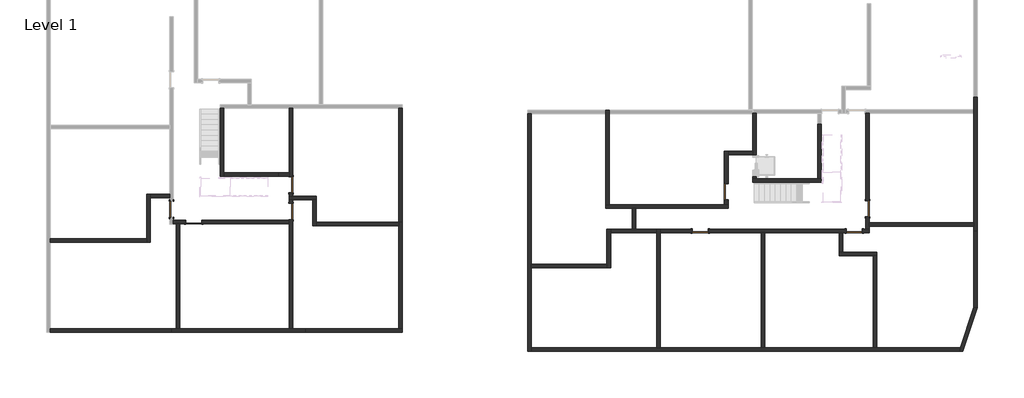
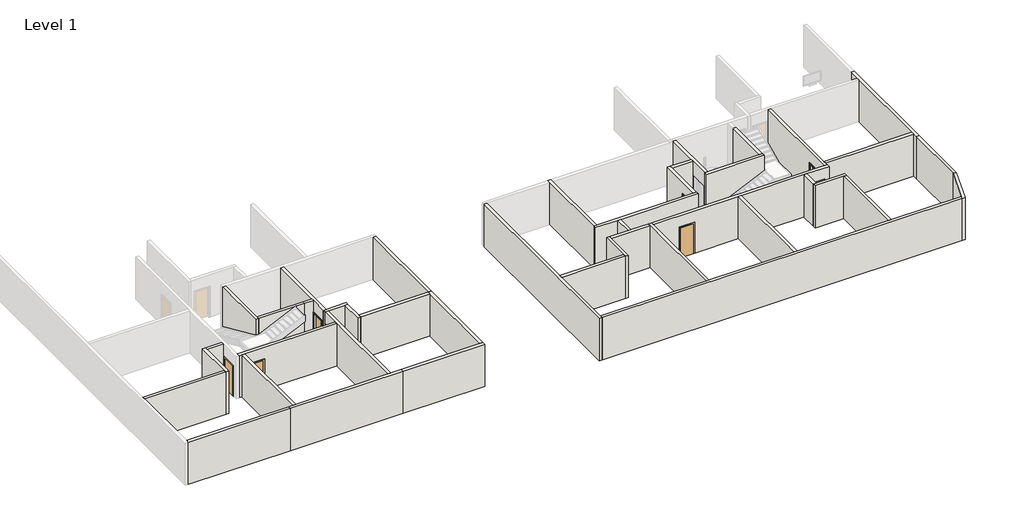
# One storey, part 1 of 2: 42 walls, 8 doors.
"""IFC4 building model written with IfcOpenShell, lengths in millimetres."""

import ifcopenshell
import ifcopenshell.guid

model = None  # the IFC model being written
_history = None  # IfcOwnerHistory: only IFC2X3 demands one
_inside = {}  # id of a spatial element -> (the spatial element, [elements in it])
_under = {}  # id of a project, library or spatial element -> (it, [spatial elements below it])
_declared = {}  # id of a project -> (the project, [libraries it declares])
_typed = {}  # id of a type object -> (the type object, [elements of that type])
_made_of = {}  # id of a material, layer set ... -> (it, [elements and type objects made of it])


def new_model(schema):
    """Start an empty IFC model of exactly this schema.

    Asked for "IFC4X3", IfcOpenShell would pick the latest addendum, in which some entities
    have other attributes; the version numbers below select the first issue.
    IFC2X3 requires an IfcOwnerHistory on every rooted entity: one is made here for all.
    """
    global model, _history
    if schema == "IFC4X3":
        model = ifcopenshell.file(schema_version=(4, 3, 0, 0))
    else:
        model = ifcopenshell.file(schema=schema)
    _inside.clear()
    _under.clear()
    _declared.clear()
    _typed.clear()
    _made_of.clear()
    _history = None
    if model.schema == "IFC2X3":
        org = make("IfcOrganization", Name="unknown")
        user = make(
            "IfcPersonAndOrganization",
            ThePerson=make("IfcPerson", FamilyName="unknown"),
            TheOrganization=org,
        )
        app = make(
            "IfcApplication",
            ApplicationDeveloper=org,
            Version="unknown",
            ApplicationFullName="unknown",
            ApplicationIdentifier="unknown",
        )
        _history = make(
            "IfcOwnerHistory",
            OwningUser=user,
            OwningApplication=app,
            ChangeAction="ADDED",
            CreationDate=0,
        )
    return model


def make(cls, **values):
    """One entity of the class cls with the attributes given. An attribute that is None is left unset."""
    return model.create_entity(
        cls, **{name: value for name, value in values.items() if value is not None}
    )


def rooted(cls, **values):
    """An entity with a GlobalId (a new one), such as an element, a storey or a relation."""
    return make(cls, GlobalId=ifcopenshell.guid.new(), OwnerHistory=_history, **values)


def si_unit(unit_type, name, prefix=None):
    """IfcSIUnit, for example si_unit("LENGTHUNIT", "METRE", prefix="MILLI")."""
    return make("IfcSIUnit", UnitType=unit_type, Prefix=prefix, Name=name)


def assignment(units):
    """IfcUnitAssignment: the units of a project."""
    return None if units is None else make("IfcUnitAssignment", Units=units)


def point(xyz):
    """IfcCartesianPoint."""
    return None if xyz is None else make("IfcCartesianPoint", Coordinates=xyz)


def direction(xyz):
    """IfcDirection."""
    return None if xyz is None else make("IfcDirection", DirectionRatios=xyz)


def frame(location, z_axis=None, x_axis=None):
    """IfcAxis2Placement3D, a coordinate frame: its origin and axes. An axis left out is left unset."""
    return make(
        "IfcAxis2Placement3D",
        Location=point(location),
        Axis=direction(z_axis),
        RefDirection=direction(x_axis),
    )


def origin():
    """The frame at (0, 0, 0) with its axes left unset."""
    return frame((0.0, 0.0, 0.0))


def origin_with_axes():
    """The frame at (0, 0, 0) with the z axis (0, 0, 1) and the x axis (1, 0, 0) written out."""
    return frame((0.0, 0.0, 0.0), z_axis=(0.0, 0.0, 1.0), x_axis=(1.0, 0.0, 0.0))


def place(relative_to, where):
    """IfcLocalPlacement: puts the frame where relative to a parent placement (None: the world)."""
    return make(
        "IfcLocalPlacement", PlacementRelTo=relative_to, RelativePlacement=where
    )


def context(
    kind, dimensions, precision=None, world=None, true_north=None, identifier=None
):
    """IfcGeometricRepresentationContext, for example the 3D "Model" context."""
    return make(
        "IfcGeometricRepresentationContext",
        ContextIdentifier=identifier,
        ContextType=kind,
        CoordinateSpaceDimension=dimensions,
        Precision=precision,
        WorldCoordinateSystem=world,
        TrueNorth=true_north,
    )


def project(units=None, contexts=None):
    """IfcProject with its units and contexts."""
    return rooted(
        "IfcProject",
        Name="project",
        RepresentationContexts=contexts,
        UnitsInContext=assignment(units),
    )


def spatial(cls, under=None, at=None, **own):
    """A site, building, storey or space (cls), placed at a placement, below another one or the project."""
    s = rooted(cls, ObjectPlacement=at, **own)
    if under is not None:
        _under.setdefault(under.id(), (under, []))[1].append(s)
    return s


def polyline(points):
    """IfcPolyline through the points."""
    return make("IfcPolyline", Points=[point(p) for p in points])


def outline(outer, holes=None, kind="AREA"):
    """IfcArbitraryClosedProfileDef: a profile drawn as a closed curve; with holes, ...WithVoids."""
    if holes is None:
        return make("IfcArbitraryClosedProfileDef", ProfileType=kind, OuterCurve=outer)
    return make(
        "IfcArbitraryProfileDefWithVoids",
        ProfileType=kind,
        OuterCurve=outer,
        InnerCurves=holes,
    )


def extrude(swept, where, along, depth):
    """IfcExtrudedAreaSolid: the profile swept, set in the frame where, extruded along a direction by depth."""
    return make(
        "IfcExtrudedAreaSolid",
        SweptArea=swept,
        Position=where,
        ExtrudedDirection=direction(along),
        Depth=depth,
    )


def faces_of(points, faces, orient=None, outer=None):
    """IfcFace entities. A face is a list of loops; a loop is a list of indices into points, from 0.

    orient and outer hold one flag for each loop. By default every Orientation is true, the
    first loop of a face is its IfcFaceOuterBound and the others are IfcFaceBound.
    """
    made = []
    for i, loops in enumerate(faces):
        bounds = []
        for j, loop in enumerate(loops):
            is_outer = j == 0 if outer is None else outer[i][j]
            bounds.append(
                make(
                    "IfcFaceOuterBound" if is_outer else "IfcFaceBound",
                    Bound=make("IfcPolyLoop", Polygon=[points[k] for k in loop]),
                    Orientation=True if orient is None else orient[i][j],
                )
            )
        made.append(make("IfcFace", Bounds=bounds))
    return made


def faceted_brep(points, faces, orient=None, outer=None, voids=None):
    """IfcFacetedBrep: a solid bounded by flat faces; with voids (closed shells), ...WithVoids."""
    shared = [point(p) for p in points]
    hull = make("IfcClosedShell", CfsFaces=faces_of(shared, faces, orient, outer))
    if voids is None:
        return make("IfcFacetedBrep", Outer=hull)
    return make(
        "IfcFacetedBrepWithVoids",
        Outer=hull,
        Voids=[
            make(cls, CfsFaces=faces_of(shared, fs, o, b)) for cls, fs, o, b in voids
        ],
    )


def shape(context_of_items, identifier, shape_type, items):
    """IfcShapeRepresentation: the items that make up one representation, for example the "Body"."""
    return make(
        "IfcShapeRepresentation",
        ContextOfItems=context_of_items,
        RepresentationIdentifier=identifier,
        RepresentationType=shape_type,
        Items=items,
    )


def source(mapping_origin, context_of_items, identifier, shape_type, items):
    """IfcRepresentationMap: a shape defined once, which mapped items show again and again."""
    return make(
        "IfcRepresentationMap",
        MappingOrigin=mapping_origin,
        MappedRepresentation=shape(context_of_items, identifier, shape_type, items),
    )


def transform(
    local_origin,
    x_axis=None,
    y_axis=None,
    z_axis=None,
    scale=None,
    scale2=None,
    scale3=None,
    uniform=True,
):
    """IfcCartesianTransformationOperator3D, or its non-uniform kind. x_axis, y_axis, z_axis: its Axis1, 2, 3."""
    if uniform:
        return make(
            "IfcCartesianTransformationOperator3D",
            Axis1=direction(x_axis),
            Axis2=direction(y_axis),
            LocalOrigin=point(local_origin),
            Scale=scale,
            Axis3=direction(z_axis),
        )
    return make(
        "IfcCartesianTransformationOperator3DnonUniform",
        Axis1=direction(x_axis),
        Axis2=direction(y_axis),
        LocalOrigin=point(local_origin),
        Scale=scale,
        Axis3=direction(z_axis),
        Scale2=scale2,
        Scale3=scale3,
    )


def mapped(mapping_source, mapping_target):
    """IfcMappedItem: shows the shape of a source again, moved by a transform."""
    return make(
        "IfcMappedItem", MappingSource=mapping_source, MappingTarget=mapping_target
    )


def made_of(thing, what):
    """Note that an element or type object is made of a material, layer set ...; save() writes the relation."""
    if what is not None:
        _made_of.setdefault(what.id(), (what, []))[1].append(thing)
    return thing


def element(
    cls,
    number,
    at=None,
    inside=None,
    cuts=None,
    type_object=None,
    material=None,
    context=None,
    identifier="Body",
    shape_type=None,
    held_by="IfcProductDefinitionShape",
    body=None,
    shapes=None,
    **own,
):
    """One element of the class cls, such as IfcWall. Its Tag is "e" and its number.

    at: its placement. inside: the storey or other place that contains it. cuts: it is an
    opening in that element (IfcRelVoidsElement). A single representation is given by context,
    identifier, shape_type and body (its items); several are given by shapes. held_by: the class
    of the entity that holds the representations. save() writes the other relations.
    """
    e = rooted(cls, Tag="e%d" % number, ObjectPlacement=at, **own)
    if body is not None:
        shapes = [shape(context, identifier, shape_type, body)]
    if shapes is not None:
        e.Representation = make(held_by, Representations=shapes)
    if inside is not None:
        _inside.setdefault(inside.id(), (inside, []))[1].append(e)
    if cuts is not None:
        rooted(
            "IfcRelVoidsElement", RelatingBuildingElement=cuts, RelatedOpeningElement=e
        )
    if type_object is not None:
        _typed.setdefault(type_object.id(), (type_object, []))[1].append(e)
    return made_of(e, material)


def aggregate(whole, parts):
    """IfcRelAggregates: a whole, such as a stair, and the parts it consists of."""
    return rooted("IfcRelAggregates", RelatingObject=whole, RelatedObjects=parts)


def save(model, path):
    """Write the relations noted so far, then the file.

    IfcRelAggregates (storeys below a building ...), IfcRelContainedInSpatialStructure (elements
    in a storey), IfcRelDefinesByType, IfcRelAssociatesMaterial and IfcRelDeclares: one each for
    every whole, place, type object, material and project.
    """
    for whole, parts in _under.values():
        aggregate(whole, parts)
    for where, things in _inside.values():
        rooted(
            "IfcRelContainedInSpatialStructure",
            RelatedElements=things,
            RelatingStructure=where,
        )
    for kind, things in _typed.values():
        rooted("IfcRelDefinesByType", RelatedObjects=things, RelatingType=kind)
    for what, things in _made_of.values():
        rooted("IfcRelAssociatesMaterial", RelatedObjects=things, RelatingMaterial=what)
    for by, libraries in _declared.values():
        rooted("IfcRelDeclares", RelatingContext=by, RelatedDefinitions=libraries)
    model.write(path)


def m_single_flush_0915_x_2134mm_727434cd(model_context):
    return source(origin(), model_context, "Body", "SweptSolid", [
        extrude(outline(polyline([(2210.0, -533.5), (0.0, -533.5), (0.0, -457.5), (2134.0, -457.5), (2134.0, 457.5), (0.0, 457.5), (0.0, 533.5), (2210.0, 533.5), (2210.0, -533.5)])), frame((0.0, -125.0, 0.0), z_axis=(0.0, 1.0, 0.0), x_axis=(0.0, 0.0, 1.0)), (0.0, 0.0, 1.0), 25.0),
        extrude(outline(polyline([(2210.0, 533.5), (2210.0, -533.5), (0.0, -533.5), (0.0, -457.5), (2134.0, -457.5), (2134.0, 457.5), (0.0, 457.5), (0.0, 533.5), (2210.0, 533.5)])), frame((0.0, 100.0, 0.0), z_axis=(0.0, 1.0, 0.0), x_axis=(0.0, 0.0, 1.0)), (0.0, 0.0, 1.0), 25.0),
        extrude(outline(polyline([(457.5, -49.0), (457.5, -100.0), (-457.5, -100.0), (-457.5, -49.0), (457.5, -49.0)])), origin_with_axes(), (0.0, 0.0, 1.0), 2134.0),
    ])


def m_single_flush_0915_x_2134mm_6a9e8738(model_context):
    return source(origin(), model_context, "Body", "SweptSolid", [
        extrude(outline(polyline([(2210.0, -533.5), (0.0, -533.5), (0.0, -457.5), (2134.0, -457.5), (2134.0, 457.5), (0.0, 457.5), (0.0, 533.5), (2210.0, 533.5), (2210.0, -533.5)])), frame((0.0, 100.0, 0.0), z_axis=(0.0, 1.0, 0.0), x_axis=(0.0, 0.0, 1.0)), (0.0, 0.0, 1.0), 25.0),
        extrude(outline(polyline([(2210.0, 533.5), (2210.0, -533.5), (0.0, -533.5), (0.0, -457.5), (2134.0, -457.5), (2134.0, 457.5), (0.0, 457.5), (0.0, 533.5), (2210.0, 533.5)])), frame((0.0, -125.0, 0.0), z_axis=(0.0, 1.0, 0.0), x_axis=(0.0, 0.0, 1.0)), (0.0, 0.0, 1.0), 25.0),
        extrude(outline(polyline([(457.5, 49.0), (-457.5, 49.0), (-457.5, 100.0), (457.5, 100.0), (457.5, 49.0)])), origin_with_axes(), (0.0, 0.0, 1.0), 2134.0),
    ])


model = new_model("IFC4")

# Units and contexts
model_context = context("Model", 3, world=origin())
ifc_project = project(units=[si_unit("LENGTHUNIT", "METRE", prefix="MILLI")], contexts=[model_context])

# Site, building, storey
site = spatial("IfcSite", under=ifc_project)
building = spatial("IfcBuilding", under=site)
storey = spatial("IfcBuildingStorey", under=building, Name="Level 1", Elevation=0.0)

# Doors
placement = place(None, origin())
m_single_flush_0915_x_2134mm_shape = m_single_flush_0915_x_2134mm_727434cd(model_context)
element("IfcDoor", 1, ObjectType="M_Single-Flush : 0915 x 2134mm", at=placement, inside=storey, context=model_context, shape_type="MappedRepresentation", body=[
    mapped(m_single_flush_0915_x_2134mm_shape, transform((16070.6041014, -3023.024372, 0.0), x_axis=(0.0, -1.0, 0.0), y_axis=(1.0, 0.0, 0.0), z_axis=(0.0, 0.0, 1.0))),
])
element("IfcDoor", 2, ObjectType="M_Single-Flush : 0915 x 2134mm", at=placement, inside=storey, context=model_context, shape_type="MappedRepresentation", body=[
    mapped(m_single_flush_0915_x_2134mm_shape, transform((-8530.3449834, -4137.6378151, 0.0), x_axis=(0.0, 1.0, 0.0), y_axis=(-1.0, 0.0, 0.0), z_axis=(0.0, 0.0, 1.0))),
])
m_single_flush_0915_x_2134mm_2_shape = m_single_flush_0915_x_2134mm_6a9e8738(model_context)
element("IfcDoor", 3, ObjectType="M_Single-Flush : 0915 x 2134mm", at=placement, inside=storey, context=model_context, shape_type="MappedRepresentation", body=[
    mapped(m_single_flush_0915_x_2134mm_2_shape, transform((14602.336337, -5240.0098119, 0.0), x_axis=(-1.0, 0.0, 0.0), y_axis=(0.0, -1.0, 0.0), z_axis=(0.0, 0.0, 1.0))),
])
element("IfcDoor", 4, ObjectType="M_Single-Flush : 0915 x 2134mm", at=placement, inside=storey, context=model_context, shape_type="MappedRepresentation", body=[
    mapped(m_single_flush_0915_x_2134mm_2_shape, transform((24048.8612349, -3982.5098119, 0.0), x_axis=(0.0, -1.0, 0.0), y_axis=(1.0, 0.0, 0.0), z_axis=(0.0, 0.0, 1.0))),
])
element("IfcDoor", 5, ObjectType="M_Single-Flush : 0915 x 2134mm", at=placement, inside=storey, context=model_context, shape_type="MappedRepresentation", body=[
    mapped(m_single_flush_0915_x_2134mm_2_shape, transform((23308.8612349, -5240.0098119, 0.0), x_axis=(-1.0, 0.0, 0.0), y_axis=(0.0, -1.0, 0.0), z_axis=(0.0, 0.0, 1.0))),
])
element("IfcDoor", 6, ObjectType="M_Single-Flush : 0915 x 2134mm", at=placement, inside=storey, context=model_context, shape_type="MappedRepresentation", body=[
    mapped(m_single_flush_0915_x_2134mm_2_shape, transform((-14032.3304233, -4739.1627129, 0.0), x_axis=(-1.0, 0.0, 0.0), y_axis=(0.0, -1.0, 0.0), z_axis=(0.0, 0.0, 1.0))),
])
element("IfcDoor", 7, ObjectType="M_Single-Flush : 0915 x 2134mm", at=placement, inside=storey, context=model_context, shape_type="MappedRepresentation", body=[
    mapped(m_single_flush_0915_x_2134mm_2_shape, transform((-8530.3449834, -2622.6378151, 0.0), x_axis=(0.0, -1.0, 0.0), y_axis=(1.0, 0.0, 0.0), z_axis=(0.0, 0.0, 1.0))),
])
element("IfcDoor", 8, ObjectType="M_Single-Flush : 0915 x 2134mm", at=placement, inside=storey, context=model_context, shape_type="MappedRepresentation", body=[
    mapped(m_single_flush_0915_x_2134mm_2_shape, transform((-15289.8304233, -3999.1627129, 0.0), x_axis=(0.0, 1.0, 0.0), y_axis=(-1.0, 0.0, 0.0), z_axis=(0.0, 0.0, 1.0))),
])

# Walls
element("IfcWall", 9, ObjectType="Generic - 200mm", at=placement, inside=storey, context=model_context, shape_type="Brep", body=[
    faceted_brep([(30068.8612349, 2319.475628, 0.0), (30068.8612349, 1619.475628, 0.0), (30068.8612349, 1419.475628, 0.0), (30068.8612349, -4760.0098119, 0.0), (30068.8612349, -4960.0098119, 0.0), (30068.8612349, -5240.0098119, 0.0), (30068.8612349, -5240.0098119, 3000.0), (30068.8612349, -4960.0098119, 3000.0), (30068.8612349, -4760.0098119, 3000.0), (30068.8612349, 1419.475628, 3000.0), (30068.8612349, 1619.475628, 3000.0), (30068.8612349, 2319.475628, 3000.0), (30268.8612349, 2319.475628, 0.0), (30268.8612349, 2319.475628, 3000.0), (30268.8612349, -5240.0098119, 3000.0), (30268.8612349, -5240.0098119, 0.0), (30268.3425199, 2319.475628, 0.0), (30069.3799498, -5240.0098119, 0.0), (30069.3799498, -5240.0098119, 3000.0), (30268.3425199, 2319.475628, 3000.0)], [[[0, 1, 2, 3, 4, 5, 6, 7, 8, 9, 10, 11]], [[12, 13, 14, 15]], [[5, 4, 3, 2, 1, 0, 16, 12, 15, 17]], [[6, 5, 17, 15, 14, 18]], [[11, 10, 9, 8, 7, 6, 18, 14, 13, 19]], [[0, 11, 19, 13, 12, 16]]]),
])
element("IfcWall", 10, ObjectType="Generic - 200mm", at=placement, inside=storey, context=model_context, shape_type="Brep", body=[
    faceted_brep([(30069.3799498, -5240.0098119, 0.0), (30069.3799498, -9543.0251929, 0.0), (30069.3799498, -9543.0251929, 3000.0), (30069.3799498, -5240.0098119, 3000.0), (30269.3799498, -5240.0098119, 0.0), (30269.3799498, -5240.0098119, 3000.0), (30269.3799498, -9575.863443, 3000.0), (30269.3799498, -9575.863443, 0.0), (30268.8612349, -5240.0098119, 0.0), (30268.8612349, -5240.0098119, 3000.0)], [[[0, 1, 2, 3]], [[4, 5, 6, 7]], [[1, 0, 8, 4, 7]], [[3, 2, 6, 5, 9]], [[0, 3, 9, 5, 4, 8]], [[2, 1, 7, 6]]]),
])
element("IfcWall", 11, ObjectType="Generic - 200mm", at=placement, inside=storey, context=model_context, shape_type="Brep", body=[
    faceted_brep([(21449.836337, -2276.2808257, 0.0), (21249.836337, -2276.2808257, 0.0), (17770.6041014, -2276.2808257, 0.0), (17570.6041014, -2276.2808257, 0.0), (17570.6041014, -2276.2808257, 3000.0), (17770.6041014, -2276.2808257, 3000.0), (21249.836337, -2276.2808257, 3000.0), (21449.836337, -2276.2808257, 3000.0), (21449.836337, -2476.2808257, 0.0), (21449.836337, -2476.2808257, 3000.0), (17570.6041014, -2476.2808257, 3000.0), (17570.6041014, -2476.2808257, 0.0)], [[[0, 1, 2, 3, 4, 5, 6, 7]], [[8, 9, 10, 11]], [[3, 2, 1, 0, 8, 11]], [[7, 6, 5, 4, 10, 9]], [[0, 7, 9, 8]], [[4, 3, 11, 10]]]),
])
element("IfcWall", 12, ObjectType="Generic - 200mm", at=placement, inside=storey, context=model_context, shape_type="SweptSolid", body=[
    extrude(outline(polyline([(18259.836337, -5340.0098119), (18259.836337, -11836.6907835), (18059.836337, -11836.6907835), (18059.836337, -5340.0098119), (18259.836337, -5340.0098119)])), origin_with_axes(), (0.0, 0.0, 1.0), 3000.0),
])
element("IfcWall", 13, ObjectType="Generic - 200mm", at=placement, inside=storey, context=model_context, shape_type="Brep", body=[
    faceted_brep([(29295.3124022, -11836.6907835, 0.0), (24588.8612349, -11836.6907835, 0.0), (24388.8612349, -11836.6907835, 0.0), (18259.836337, -11836.6907835, 0.0), (18059.836337, -11836.6907835, 0.0), (12342.1281129, -11836.6907835, 0.0), (12142.1281129, -11836.6907835, 0.0), (5043.716007, -11836.6907835, 0.0), (5043.716007, -11836.6907835, 3000.0), (12142.1281129, -11836.6907835, 3000.0), (12342.1281129, -11836.6907835, 3000.0), (18059.836337, -11836.6907835, 3000.0), (18259.836337, -11836.6907835, 3000.0), (24388.8612349, -11836.6907835, 3000.0), (24588.8612349, -11836.6907835, 3000.0), (29295.3124022, -11836.6907835, 3000.0), (29227.8162902, -12036.6907835, 0.0), (29227.8162902, -12036.6907835, 3000.0), (5043.716007, -12036.6907835, 3000.0), (5043.716007, -12036.6907835, 0.0)], [[[0, 1, 2, 3, 4, 5, 6, 7, 8, 9, 10, 11, 12, 13, 14, 15]], [[16, 17, 18, 19]], [[7, 6, 5, 4, 3, 2, 1, 0, 16, 19]], [[15, 14, 13, 12, 11, 10, 9, 8, 18, 17]], [[0, 15, 17, 16]], [[8, 7, 19, 18]]]),
])
element("IfcWall", 14, ObjectType="Generic - 200mm", at=placement, inside=storey, context=model_context, shape_type="Brep", body=[
    faceted_brep([(30069.3799498, -9543.0251929, 0.0), (29295.3124022, -11836.6907835, 0.0), (29227.8162902, -12036.6907835, 0.0), (29227.8162902, -12036.6907835, 3000.0), (29295.3124022, -11836.6907835, 3000.0), (30069.3799498, -9543.0251929, 3000.0), (30269.3799498, -9575.863443, 0.0), (30269.3799498, -9575.863443, 3000.0), (29438.8985612, -12036.6907835, 3000.0), (29438.8985612, -12036.6907835, 0.0)], [[[0, 1, 2, 3, 4, 5]], [[6, 7, 8, 9]], [[2, 1, 0, 6, 9]], [[5, 4, 3, 8, 7]], [[0, 5, 7, 6]], [[3, 2, 9, 8]]]),
])
element("IfcWall", 15, ObjectType="Generic - 200mm", at=placement, inside=storey, context=model_context, shape_type="Brep", body=[
    faceted_brep([(22851.3612349, -5140.0098119, 2134.0), (22851.3612349, -5140.0098119, 0.0), (15059.836337, -5140.0098119, 0.0), (15059.836337, -5140.0098119, 2134.0), (14144.836337, -5140.0098119, 2134.0), (14144.836337, -5140.0098119, 0.0), (12342.1281129, -5140.0098119, 0.0), (12342.1281129, -5140.0098119, 3000.0), (23948.8612349, -5140.0098119, 3000.0), (24148.8612349, -5140.0098119, 3000.0), (24163.3998354, -5140.0098119, 3000.0), (24163.3998354, -5140.0098119, 0.0), (24148.8612349, -5140.0098119, 0.0), (23948.8612349, -5140.0098119, 0.0), (23766.3612349, -5140.0098119, 0.0), (23766.3612349, -5140.0098119, 2134.0), (15059.836337, -5340.0098119, 0.0), (18059.836337, -5340.0098119, 0.0), (18259.836337, -5340.0098119, 0.0), (22468.8612349, -5340.0098119, 0.0), (22668.8612349, -5340.0098119, 0.0), (22851.3612349, -5340.0098119, 0.0), (22851.3612349, -5340.0098119, 2134.0), (23766.3612349, -5340.0098119, 2134.0), (23766.3612349, -5340.0098119, 0.0), (24163.3998354, -5340.0098119, 0.0), (24163.3998354, -5340.0098119, 3000.0), (22668.8612349, -5340.0098119, 3000.0), (22468.8612349, -5340.0098119, 3000.0), (18259.836337, -5340.0098119, 3000.0), (18059.836337, -5340.0098119, 3000.0), (12342.1281129, -5340.0098119, 3000.0), (12342.1281129, -5340.0098119, 0.0), (14144.836337, -5340.0098119, 0.0), (14144.836337, -5340.0098119, 2134.0), (15059.836337, -5340.0098119, 2134.0)], [[[0, 1, 2, 3, 4, 5, 6, 7, 8, 9, 10, 11, 12, 13, 14, 15]], [[16, 17, 18, 19, 20, 21, 22, 23, 24, 25, 26, 27, 28, 29, 30, 31, 32, 33, 34, 35]], [[32, 6, 5, 33]], [[2, 1, 21, 20, 19, 18, 17, 16]], [[14, 13, 12, 11, 25, 24]], [[10, 9, 8, 7, 31, 30, 29, 28, 27, 26]], [[11, 10, 26, 25]], [[4, 34, 33, 5]], [[35, 3, 2, 16]], [[3, 35, 34, 4]], [[22, 21, 1, 0]], [[23, 22, 0, 15]], [[24, 23, 15, 14]], [[7, 6, 32, 31]]]),
])
element("IfcWall", 16, ObjectType="Generic - 200mm", at=placement, inside=storey, context=model_context, shape_type="Brep", body=[
    faceted_brep([(4843.716007, 1379.9901881, 0.0), (4843.716007, -12036.6907835, 0.0), (4843.716007, -12036.6907835, 3000.0), (4843.716007, 1379.9901881, 3000.0), (5043.716007, 1379.9901881, 0.0), (5043.716007, 1379.9901881, 3000.0), (5043.716007, -7120.0098119, 3000.0), (5043.716007, -7320.0098119, 3000.0), (5043.716007, -11836.6907835, 3000.0), (5043.716007, -12036.6907835, 3000.0), (5043.716007, -12036.6907835, 0.0), (5043.716007, -11836.6907835, 0.0), (5043.716007, -7320.0098119, 0.0), (5043.716007, -7120.0098119, 0.0)], [[[0, 1, 2, 3]], [[4, 5, 6, 7, 8, 9, 10, 11, 12, 13]], [[1, 0, 4, 13, 12, 11, 10]], [[3, 2, 9, 8, 7, 6, 5]], [[2, 1, 10, 9]], [[0, 3, 5, 4]]]),
])
element("IfcWall", 17, ObjectType="Generic - 200mm", at=placement, inside=storey, context=model_context, shape_type="Brep", body=[
    faceted_brep([(24148.8612349, 1419.475628, 3000.0), (24148.8612349, -4760.0098119, 3000.0), (24148.8612349, -4960.0098119, 3000.0), (24148.8612349, -5140.0098119, 3000.0), (24148.8612349, -5140.0098119, 0.0), (24148.8612349, -4960.0098119, 0.0), (24148.8612349, -4760.0098119, 0.0), (24148.8612349, -4440.0098119, 0.0), (24148.8612349, -4440.0098119, 2134.0), (24148.8612349, -3525.0098119, 2134.0), (24148.8612349, -3525.0098119, 0.0), (24148.8612349, 1419.475628, 0.0), (23948.8612349, -5140.0098119, 3000.0), (23948.8612349, 1419.475628, 3000.0), (23948.8612349, 1419.475628, 0.0), (23948.8612349, -3525.0098119, 0.0), (23948.8612349, -3525.0098119, 2134.0), (23948.8612349, -4440.0098119, 2134.0), (23948.8612349, -4440.0098119, 0.0), (23948.8612349, -5140.0098119, 0.0)], [[[0, 1, 2, 3, 4, 5, 6, 7, 8, 9, 10, 11]], [[12, 13, 14, 15, 16, 17, 18, 19]], [[14, 11, 10, 15]], [[4, 19, 18, 7, 6, 5]], [[3, 2, 1, 0, 13, 12]], [[0, 11, 14, 13]], [[17, 8, 7, 18]], [[9, 16, 15, 10]], [[16, 9, 8, 17]], [[4, 3, 12, 19]]]),
])
element("IfcWall", 18, ObjectType="Generic - 200mm", at=placement, inside=storey, context=model_context, shape_type="SweptSolid", body=[
    extrude(outline(polyline([(21249.836337, -2276.2808257), (21249.836337, 799.475628), (21449.836337, 799.475628), (21449.836337, -2276.2808257), (21249.836337, -2276.2808257)])), origin_with_axes(), (0.0, 0.0, 1.0), 3000.0),
])
element("IfcWall", 19, ObjectType="Generic - 200mm", at=placement, inside=storey, context=model_context, shape_type="Brep", body=[
    faceted_brep([(17570.6041014, -2276.2808257, 3000.0), (17570.6041014, -920.524372, 3000.0), (17570.6041014, -720.524372, 3000.0), (17570.6041014, 1379.475628, 3000.0), (17570.6041014, 1419.475628, 3000.0), (17570.6041014, 1419.475628, 0.0), (17570.6041014, 1379.475628, 0.0), (17570.6041014, -720.524372, 0.0), (17570.6041014, -920.524372, 0.0), (17570.6041014, -926.2808257, 0.0), (17570.6041014, -926.2808257, 2000.0), (17570.6041014, -2181.2876228, 2000.0), (17570.6041014, -2181.2876228, 0.0), (17570.6041014, -2276.2808257, 0.0), (17770.6041014, 1419.475628, 3000.0), (17770.6041014, -2276.2808257, 3000.0), (17770.6041014, -2276.2808257, 0.0), (17770.6041014, -2181.2876228, 0.0), (17770.6041014, -2181.2876228, 2000.0), (17770.6041014, -926.2808257, 2000.0), (17770.6041014, -926.2808257, 0.0), (17770.6041014, 1419.475628, 0.0)], [[[0, 1, 2, 3, 4, 5, 6, 7, 8, 9, 10, 11, 12, 13]], [[14, 15, 16, 17, 18, 19, 20, 21]], [[16, 13, 12, 17]], [[5, 21, 20, 9, 8, 7, 6]], [[4, 3, 2, 1, 0, 15, 14]], [[0, 13, 16, 15]], [[5, 4, 14, 21]], [[11, 18, 17, 12]], [[19, 10, 9, 20]], [[10, 19, 18, 11]]]),
])
element("IfcWall", 20, ObjectType="Generic - 200mm", at=placement, inside=storey, context=model_context, shape_type="Brep", body=[
    faceted_brep([(9268.8612349, -3940.0098119, 0.0), (10768.8612349, -3940.0098119, 0.0), (10968.8612349, -3940.0098119, 0.0), (16170.6041014, -3940.0098119, 0.0), (16170.6041014, -3940.0098119, 3000.0), (10968.8612349, -3940.0098119, 3000.0), (10768.8612349, -3940.0098119, 3000.0), (9268.8612349, -3940.0098119, 3000.0), (9268.8612349, -3740.0098119, 0.0), (9268.8612349, -3740.0098119, 3000.0), (9468.8612349, -3740.0098119, 3000.0), (15970.6041014, -3740.0098119, 3000.0), (16170.6041014, -3740.0098119, 3000.0), (16170.6041014, -3740.0098119, 0.0), (15970.6041014, -3740.0098119, 0.0), (9468.8612349, -3740.0098119, 0.0)], [[[0, 1, 2, 3, 4, 5, 6, 7]], [[8, 9, 10, 11, 12, 13, 14, 15]], [[3, 2, 1, 0, 8, 15, 14, 13]], [[7, 6, 5, 4, 12, 11, 10, 9]], [[4, 3, 13, 12]], [[0, 7, 9, 8]]]),
])
element("IfcWall", 21, ObjectType="Generic - 200mm", at=placement, inside=storey, context=model_context, shape_type="Brep", body=[
    faceted_brep([(16170.6041014, -720.524372, 3000.0), (16170.6041014, -920.524372, 3000.0), (16170.6041014, -3740.0098119, 3000.0), (16170.6041014, -3740.0098119, 0.0), (16170.6041014, -3480.524372, 0.0), (16170.6041014, -3480.524372, 2134.0), (16170.6041014, -2565.524372, 2134.0), (16170.6041014, -2565.524372, 0.0), (16170.6041014, -920.524372, 0.0), (16170.6041014, -720.524372, 0.0), (15970.6041014, -3740.0098119, 3000.0), (15970.6041014, -720.524372, 3000.0), (15970.6041014, -720.524372, 0.0), (15970.6041014, -2565.524372, 0.0), (15970.6041014, -2565.524372, 2134.0), (15970.6041014, -3480.524372, 2134.0), (15970.6041014, -3480.524372, 0.0), (15970.6041014, -3740.0098119, 0.0)], [[[0, 1, 2, 3, 4, 5, 6, 7, 8, 9]], [[10, 11, 12, 13, 14, 15, 16, 17]], [[3, 17, 16, 4]], [[12, 9, 8, 7, 13]], [[2, 1, 0, 11, 10]], [[3, 2, 10, 17]], [[0, 9, 12, 11]], [[15, 5, 4, 16]], [[6, 14, 13, 7]], [[14, 6, 5, 15]]]),
])
element("IfcWall", 22, ObjectType="Generic - 200mm", at=placement, inside=storey, context=model_context, shape_type="SweptSolid", body=[
    extrude(outline(polyline([(17570.6041014, -920.524372), (16170.6041014, -920.524372), (16170.6041014, -720.524372), (17570.6041014, -720.524372), (17570.6041014, -920.524372)])), origin_with_axes(), (0.0, 0.0, 1.0), 3000.0),
])
element("IfcWall", 23, ObjectType="Generic - 200mm", at=placement, inside=storey, context=model_context, shape_type="Brep", body=[
    faceted_brep([(22468.8612349, -6641.2808257, 0.0), (24388.8612349, -6641.2808257, 0.0), (24588.8612349, -6641.2808257, 0.0), (24588.8612349, -6641.2808257, 3000.0), (24388.8612349, -6641.2808257, 3000.0), (22468.8612349, -6641.2808257, 3000.0), (22468.8612349, -6441.2808257, 0.0), (22468.8612349, -6441.2808257, 3000.0), (22668.8612349, -6441.2808257, 3000.0), (24588.8612349, -6441.2808257, 3000.0), (24588.8612349, -6441.2808257, 0.0), (22668.8612349, -6441.2808257, 0.0)], [[[0, 1, 2, 3, 4, 5]], [[6, 7, 8, 9, 10, 11]], [[2, 1, 0, 6, 11, 10]], [[5, 4, 3, 9, 8, 7]], [[3, 2, 10, 9]], [[0, 5, 7, 6]]]),
])
element("IfcWall", 24, ObjectType="Generic - 200mm", at=placement, inside=storey, context=model_context, shape_type="SweptSolid", body=[
    extrude(outline(polyline([(24388.8612349, -11836.6907835), (24388.8612349, -6641.2808257), (24588.8612349, -6641.2808257), (24588.8612349, -11836.6907835), (24388.8612349, -11836.6907835)])), origin_with_axes(), (0.0, 0.0, 1.0), 3000.0),
])
element("IfcWall", 25, ObjectType="Generic - 200mm", at=placement, inside=storey, context=model_context, shape_type="SweptSolid", body=[
    extrude(outline(polyline([(22668.8612349, -5340.0098119), (22668.8612349, -6441.2808257), (22468.8612349, -6441.2808257), (22468.8612349, -5340.0098119), (22668.8612349, -5340.0098119)])), origin_with_axes(), (0.0, 0.0, 1.0), 3000.0),
])
element("IfcWall", 26, ObjectType="Generic - 200mm", at=placement, inside=storey, context=model_context, shape_type="SweptSolid", body=[
    extrude(outline(polyline([(30068.8612349, -4960.0098119), (24148.8612349, -4960.0098119), (24148.8612349, -4760.0098119), (30068.8612349, -4760.0098119), (30068.8612349, -4960.0098119)])), origin_with_axes(), (0.0, 0.0, 1.0), 3000.0),
])
element("IfcWall", 27, ObjectType="Generic - 200mm", at=placement, inside=storey, context=model_context, shape_type="Brep", body=[
    faceted_brep([(9268.8612349, 1579.9901881, 0.0), (9268.8612349, 1379.9901881, 0.0), (9268.8612349, -3740.0098119, 0.0), (9268.8612349, -3740.0098119, 3000.0), (9268.8612349, 1379.9901881, 3000.0), (9268.8612349, 1579.9901881, 3000.0), (9468.8612349, 1579.9901881, 0.0), (9468.8612349, 1579.9901881, 3000.0), (9468.8612349, 1579.475628, 3000.0), (9468.8612349, 1379.475628, 3000.0), (9468.8612349, -3740.0098119, 3000.0), (9468.8612349, -3740.0098119, 0.0), (9468.8612349, 1379.475628, 0.0), (9468.8612349, 1579.475628, 0.0)], [[[0, 1, 2, 3, 4, 5]], [[6, 7, 8, 9, 10, 11, 12, 13]], [[2, 1, 0, 6, 13, 12, 11]], [[5, 4, 3, 10, 9, 8, 7]], [[3, 2, 11, 10]], [[0, 5, 7, 6]]]),
])
element("IfcWall", 28, ObjectType="Generic - 200mm", at=placement, inside=storey, context=model_context, shape_type="SweptSolid", body=[
    extrude(outline(polyline([(5043.716007, -7120.0098119), (9328.8612349, -7120.0098119), (9328.8612349, -7320.0098119), (5043.716007, -7320.0098119), (5043.716007, -7120.0098119)])), origin_with_axes(), (0.0, 0.0, 1.0), 3000.0),
])
element("IfcWall", 29, ObjectType="Generic - 200mm", at=placement, inside=storey, context=model_context, shape_type="Brep", body=[
    faceted_brep([(-2430.3449834, -4740.1378151, 0.0), (-2430.3449834, -4940.1378151, 0.0), (-2430.3449834, -10758.643998, 0.0), (-2430.3449834, -10758.643998, 3000.0), (-2430.3449834, -4940.1378151, 3000.0), (-2430.3449834, -4740.1378151, 3000.0), (-2230.3449834, -4740.1378151, 0.0), (-2230.3449834, -4740.1378151, 3000.0), (-2230.3449834, -10758.643998, 3000.0), (-2230.3449834, -10758.643998, 0.0)], [[[0, 1, 2, 3, 4, 5]], [[6, 7, 8, 9]], [[2, 1, 0, 6, 9]], [[5, 4, 3, 8, 7]], [[3, 2, 9, 8]], [[0, 5, 7, 6]]]),
])
element("IfcWall", 30, ObjectType="Generic - 200mm", at=placement, inside=storey, context=model_context, shape_type="Brep", body=[
    faceted_brep([(-2230.3449834, -10758.643998, 0.0), (-2430.3449834, -10758.643998, 0.0), (-7730.3449834, -10758.643998, 0.0), (-7730.3449834, -10758.643998, 3000.0), (-2430.3449834, -10758.643998, 3000.0), (-2230.3449834, -10758.643998, 3000.0), (-2230.3449834, -10958.643998, 0.0), (-2230.3449834, -10958.643998, 3000.0), (-7730.3449834, -10958.643998, 3000.0), (-7730.3449834, -10958.643998, 0.0), (-7730.3449834, -10759.1627129, 0.0), (-7730.3449834, -10759.1627129, 3000.0)], [[[0, 1, 2, 3, 4, 5]], [[6, 7, 8, 9]], [[2, 1, 0, 6, 9, 10]], [[3, 2, 10, 9, 8, 11]], [[5, 4, 3, 11, 8, 7]], [[0, 5, 7, 6]]]),
])
element("IfcWall", 31, ObjectType="Generic - 200mm", at=placement, inside=storey, context=model_context, shape_type="Brep", body=[
    faceted_brep([(-7730.3449834, -10759.1627129, 0.0), (-8430.3449834, -10759.1627129, 0.0), (-8630.3449834, -10759.1627129, 0.0), (-14809.8304233, -10759.1627129, 0.0), (-15009.8304233, -10759.1627129, 0.0), (-15289.8304233, -10759.1627129, 0.0), (-15289.8304233, -10759.1627129, 3000.0), (-15009.8304233, -10759.1627129, 3000.0), (-14809.8304233, -10759.1627129, 3000.0), (-8630.3449834, -10759.1627129, 3000.0), (-8430.3449834, -10759.1627129, 3000.0), (-7730.3449834, -10759.1627129, 3000.0), (-7730.3449834, -10959.1627129, 0.0), (-7730.3449834, -10959.1627129, 3000.0), (-15289.8304233, -10959.1627129, 3000.0), (-15289.8304233, -10959.1627129, 0.0), (-7730.3449834, -10958.643998, 0.0), (-15289.8304233, -10759.6814279, 0.0), (-15289.8304233, -10759.6814279, 3000.0), (-7730.3449834, -10958.643998, 3000.0)], [[[0, 1, 2, 3, 4, 5, 6, 7, 8, 9, 10, 11]], [[12, 13, 14, 15]], [[5, 4, 3, 2, 1, 0, 16, 12, 15, 17]], [[6, 5, 17, 15, 14, 18]], [[11, 10, 9, 8, 7, 6, 18, 14, 13, 19]], [[0, 11, 19, 13, 12, 16]]]),
])
element("IfcWall", 32, ObjectType="Generic - 200mm", at=placement, inside=storey, context=model_context, shape_type="Brep", body=[
    faceted_brep([(-15289.8304233, -10759.6814279, 0.0), (-22146.5113948, -10759.6814279, 0.0), (-22146.5113948, -10759.6814279, 3000.0), (-15289.8304233, -10759.6814279, 3000.0), (-15289.8304233, -10959.6814279, 0.0), (-15289.8304233, -10959.6814279, 3000.0), (-22146.5113948, -10959.6814279, 3000.0), (-22146.5113948, -10959.6814279, 0.0), (-15289.8304233, -10959.1627129, 0.0), (-15289.8304233, -10959.1627129, 3000.0)], [[[0, 1, 2, 3]], [[4, 5, 6, 7]], [[1, 0, 8, 4, 7]], [[3, 2, 6, 5, 9]], [[0, 3, 9, 5, 4, 8]], [[2, 1, 7, 6]]]),
])
element("IfcWall", 33, ObjectType="Generic - 200mm", at=placement, inside=storey, context=model_context, shape_type="Brep", body=[
    faceted_brep([(-12326.101437, -2140.1378151, 0.0), (-12326.101437, -1940.1378151, 0.0), (-12326.101437, 1699.0944206, 0.0), (-12326.101437, 1699.0944206, 3000.0), (-12326.101437, -1940.1378151, 3000.0), (-12326.101437, -2140.1378151, 3000.0), (-12526.101437, -2140.1378151, 0.0), (-12526.101437, -2140.1378151, 3000.0), (-12526.101437, 1699.0944206, 3000.0), (-12526.101437, 1699.0944206, 0.0)], [[[0, 1, 2, 3, 4, 5]], [[6, 7, 8, 9]], [[2, 1, 0, 6, 9]], [[3, 2, 9, 8]], [[5, 4, 3, 8, 7]], [[0, 5, 7, 6]]]),
])
element("IfcWall", 34, ObjectType="Generic - 200mm", at=placement, inside=storey, context=model_context, shape_type="Brep", body=[
    faceted_brep([(-8630.3449834, -4839.1627129, 3000.0), (-14809.8304233, -4839.1627129, 3000.0), (-15009.8304233, -4839.1627129, 3000.0), (-15189.8304233, -4839.1627129, 3000.0), (-15189.8304233, -4839.1627129, 0.0), (-15009.8304233, -4839.1627129, 0.0), (-14809.8304233, -4839.1627129, 0.0), (-14489.8304233, -4839.1627129, 0.0), (-14489.8304233, -4839.1627129, 2134.0), (-13574.8304233, -4839.1627129, 2134.0), (-13574.8304233, -4839.1627129, 0.0), (-8630.3449834, -4839.1627129, 0.0), (-15189.8304233, -4639.1627129, 3000.0), (-8630.3449834, -4639.1627129, 3000.0), (-8630.3449834, -4639.1627129, 0.0), (-13574.8304233, -4639.1627129, 0.0), (-13574.8304233, -4639.1627129, 2134.0), (-14489.8304233, -4639.1627129, 2134.0), (-14489.8304233, -4639.1627129, 0.0), (-15189.8304233, -4639.1627129, 0.0)], [[[0, 1, 2, 3, 4, 5, 6, 7, 8, 9, 10, 11]], [[12, 13, 14, 15, 16, 17, 18, 19]], [[14, 11, 10, 15]], [[4, 19, 18, 7, 6, 5]], [[3, 2, 1, 0, 13, 12]], [[0, 11, 14, 13]], [[17, 8, 7, 18]], [[9, 16, 15, 10]], [[16, 9, 8, 17]], [[4, 3, 12, 19]]]),
])
element("IfcWall", 35, ObjectType="Generic - 200mm", at=placement, inside=storey, context=model_context, shape_type="SweptSolid", body=[
    extrude(outline(polyline([(-12326.101437, -1940.1378151), (-9250.3449834, -1940.1378151), (-9250.3449834, -2140.1378151), (-12326.101437, -2140.1378151), (-12326.101437, -1940.1378151)])), origin_with_axes(), (0.0, 0.0, 1.0), 3000.0),
])
element("IfcWall", 36, ObjectType="Generic - 200mm", at=placement, inside=storey, context=model_context, shape_type="SweptSolid", body=[
    extrude(outline(polyline([(-8630.3449834, -2140.1378151), (-9250.3449834, -2140.1378151), (-9250.3449834, -1940.1378151), (-8630.3449834, -1940.1378151), (-8630.3449834, -2140.1378151)])), origin_with_axes(), (0.0, 0.0, 1.0), 3000.0),
])
element("IfcWall", 37, ObjectType="Generic - 200mm", at=placement, inside=storey, context=model_context, shape_type="SweptSolid", body=[
    extrude(outline(polyline([(-2430.3449834, -4740.1378151), (-2430.3449834, 1700.8372871), (-2230.3449834, 1700.8372871), (-2230.3449834, -4740.1378151), (-2430.3449834, -4740.1378151)])), origin_with_axes(), (0.0, 0.0, 1.0), 3000.0),
])
element("IfcWall", 38, ObjectType="Generic - 200mm", at=placement, inside=storey, context=model_context, shape_type="Brep", body=[
    faceted_brep([(-8630.3449834, -3480.1378151, 0.0), (-8430.3449834, -3480.1378151, 0.0), (-7295.3449834, -3480.1378151, 0.0), (-7095.3449834, -3480.1378151, 0.0), (-7095.3449834, -3480.1378151, 3000.0), (-7295.3449834, -3480.1378151, 3000.0), (-8430.3449834, -3480.1378151, 3000.0), (-8630.3449834, -3480.1378151, 3000.0), (-8630.3449834, -3280.1378151, 0.0), (-8630.3449834, -3280.1378151, 3000.0), (-8430.3449834, -3280.1378151, 3000.0), (-7095.3449834, -3280.1378151, 3000.0), (-7095.3449834, -3280.1378151, 0.0), (-8430.3449834, -3280.1378151, 0.0)], [[[0, 1, 2, 3, 4, 5, 6, 7]], [[8, 9, 10, 11, 12, 13]], [[3, 2, 1, 0, 8, 13, 12]], [[7, 6, 5, 4, 11, 10, 9]], [[0, 7, 9, 8]], [[4, 3, 12, 11]]]),
])
element("IfcWall", 39, ObjectType="Generic - 200mm", at=placement, inside=storey, context=model_context, shape_type="Brep", body=[
    faceted_brep([(-8630.3449834, -10759.1627129, 3000.0), (-8630.3449834, -4839.1627129, 3000.0), (-8630.3449834, -4639.1627129, 3000.0), (-8630.3449834, -3480.1378151, 3000.0), (-8630.3449834, -3480.1378151, 0.0), (-8630.3449834, -3680.1378151, 0.0), (-8630.3449834, -3680.1378151, 2134.0), (-8630.3449834, -4595.1378151, 2134.0), (-8630.3449834, -4595.1378151, 0.0), (-8630.3449834, -4639.1627129, 0.0), (-8630.3449834, -4839.1627129, 0.0), (-8630.3449834, -10759.1627129, 0.0), (-8430.3449834, -3480.1378151, 3000.0), (-8430.3449834, -10759.1627129, 3000.0), (-8430.3449834, -10759.1627129, 0.0), (-8430.3449834, -4595.1378151, 0.0), (-8430.3449834, -4595.1378151, 2134.0), (-8430.3449834, -3680.1378151, 2134.0), (-8430.3449834, -3680.1378151, 0.0), (-8430.3449834, -3480.1378151, 0.0)], [[[0, 1, 2, 3, 4, 5, 6, 7, 8, 9, 10, 11]], [[12, 13, 14, 15, 16, 17, 18, 19]], [[14, 11, 10, 9, 8, 15]], [[4, 19, 18, 5]], [[3, 2, 1, 0, 13, 12]], [[0, 11, 14, 13]], [[4, 3, 12, 19]], [[17, 6, 5, 18]], [[7, 16, 15, 8]], [[16, 7, 6, 17]]]),
])
element("IfcWall", 40, ObjectType="Generic - 200mm", at=placement, inside=storey, context=model_context, shape_type="Brep", body=[
    faceted_brep([(-8430.3449834, 1700.8372871, 3000.0), (-8430.3449834, -3280.1378151, 3000.0), (-8430.3449834, -3280.1378151, 0.0), (-8430.3449834, -3080.1378151, 0.0), (-8430.3449834, -3080.1378151, 2134.0), (-8430.3449834, -2165.1378151, 2134.0), (-8430.3449834, -2165.1378151, 0.0), (-8430.3449834, 1700.8372871, 0.0), (-8630.3449834, -3280.1378151, 3000.0), (-8630.3449834, -2140.1378151, 3000.0), (-8630.3449834, -1940.1378151, 3000.0), (-8630.3449834, 1700.8372871, 3000.0), (-8630.3449834, 1700.8372871, 0.0), (-8630.3449834, -1940.1378151, 0.0), (-8630.3449834, -2140.1378151, 0.0), (-8630.3449834, -2165.1378151, 0.0), (-8630.3449834, -2165.1378151, 2134.0), (-8630.3449834, -3080.1378151, 2134.0), (-8630.3449834, -3080.1378151, 0.0), (-8630.3449834, -3280.1378151, 0.0)], [[[0, 1, 2, 3, 4, 5, 6, 7]], [[8, 9, 10, 11, 12, 13, 14, 15, 16, 17, 18, 19]], [[2, 19, 18, 3]], [[12, 7, 6, 15, 14, 13]], [[1, 0, 11, 10, 9, 8]], [[2, 1, 8, 19]], [[17, 4, 3, 18]], [[5, 16, 15, 6]], [[16, 5, 4, 17]], [[0, 7, 12, 11]]]),
])
element("IfcWall", 41, ObjectType="Generic - 200mm", at=placement, inside=storey, context=model_context, shape_type="Brep", body=[
    faceted_brep([(-7295.3449834, -3480.1378151, 0.0), (-7295.3449834, -4940.1378151, 0.0), (-7295.3449834, -4940.1378151, 3000.0), (-7295.3449834, -3480.1378151, 3000.0), (-7095.3449834, -3480.1378151, 0.0), (-7095.3449834, -3480.1378151, 3000.0), (-7095.3449834, -4740.1378151, 3000.0), (-7095.3449834, -4940.1378151, 3000.0), (-7095.3449834, -4940.1378151, 0.0), (-7095.3449834, -4740.1378151, 0.0)], [[[0, 1, 2, 3]], [[4, 5, 6, 7, 8, 9]], [[1, 0, 4, 9, 8]], [[3, 2, 7, 6, 5]], [[2, 1, 8, 7]], [[0, 3, 5, 4]]]),
])
element("IfcWall", 42, ObjectType="Generic - 200mm", at=placement, inside=storey, context=model_context, shape_type="SweptSolid", body=[
    extrude(outline(polyline([(-2430.3449834, -4940.1378151), (-7095.3449834, -4940.1378151), (-7095.3449834, -4740.1378151), (-2430.3449834, -4740.1378151), (-2430.3449834, -4940.1378151)])), origin_with_axes(), (0.0, 0.0, 1.0), 3000.0),
])
element("IfcWall", 43, ObjectType="Generic - 200mm", at=placement, inside=storey, context=model_context, shape_type="Brep", body=[
    faceted_brep([(-16691.101437, -3159.1627129, 0.0), (-16691.101437, -5679.1627129, 0.0), (-16691.101437, -5879.1627129, 0.0), (-16691.101437, -5879.1627129, 3000.0), (-16691.101437, -5679.1627129, 3000.0), (-16691.101437, -3159.1627129, 3000.0), (-16491.101437, -3159.1627129, 0.0), (-16491.101437, -3159.1627129, 3000.0), (-16491.101437, -3359.1627129, 3000.0), (-16491.101437, -5879.1627129, 3000.0), (-16491.101437, -5879.1627129, 0.0), (-16491.101437, -3359.1627129, 0.0)], [[[0, 1, 2, 3, 4, 5]], [[6, 7, 8, 9, 10, 11]], [[2, 1, 0, 6, 11, 10]], [[5, 4, 3, 9, 8, 7]], [[3, 2, 10, 9]], [[0, 5, 7, 6]]]),
])
element("IfcWall", 44, ObjectType="Generic - 200mm", at=placement, inside=storey, context=model_context, shape_type="SweptSolid", body=[
    extrude(outline(polyline([(-22146.5113948, -5679.1627129), (-16691.101437, -5679.1627129), (-16691.101437, -5879.1627129), (-22146.5113948, -5879.1627129), (-22146.5113948, -5679.1627129)])), origin_with_axes(), (0.0, 0.0, 1.0), 3000.0),
])
element("IfcWall", 45, ObjectType="Generic - 200mm", at=placement, inside=storey, context=model_context, shape_type="SweptSolid", body=[
    extrude(outline(polyline([(-15389.8304233, -3359.1627129), (-16491.101437, -3359.1627129), (-16491.101437, -3159.1627129), (-15389.8304233, -3159.1627129), (-15389.8304233, -3359.1627129)])), origin_with_axes(), (0.0, 0.0, 1.0), 3000.0),
])
element("IfcWall", 46, ObjectType="Generic - 200mm", at=placement, inside=storey, context=model_context, shape_type="SweptSolid", body=[
    extrude(outline(polyline([(-15009.8304233, -10759.1627129), (-15009.8304233, -4839.1627129), (-14809.8304233, -4839.1627129), (-14809.8304233, -10759.1627129), (-15009.8304233, -10759.1627129)])), origin_with_axes(), (0.0, 0.0, 1.0), 3000.0),
])
element("IfcWall", 47, ObjectType="Generic - 200mm", at=placement, inside=storey, context=model_context, shape_type="Brep", body=[
    faceted_brep([(12142.1281129, -5136.6907835, 0.0), (12142.1281129, -5336.6907835, 0.0), (12142.1281129, -11836.6907835, 0.0), (12142.1281129, -11836.6907835, 3000.0), (12142.1281129, -5336.6907835, 3000.0), (12142.1281129, -5136.6907835, 3000.0), (12342.1281129, -5136.6907835, 0.0), (12342.1281129, -5136.6907835, 3000.0), (12342.1281129, -5140.0098119, 3000.0), (12342.1281129, -5340.0098119, 3000.0), (12342.1281129, -11836.6907835, 3000.0), (12342.1281129, -11836.6907835, 0.0), (12342.1281129, -5340.0098119, 0.0), (12342.1281129, -5140.0098119, 0.0)], [[[0, 1, 2, 3, 4, 5]], [[6, 7, 8, 9, 10, 11, 12, 13]], [[2, 1, 0, 6, 13, 12, 11]], [[5, 4, 3, 10, 9, 8, 7]], [[3, 2, 11, 10]], [[0, 5, 7, 6]]]),
])
element("IfcWall", 48, ObjectType="Generic - 200mm", at=placement, inside=storey, context=model_context, shape_type="Brep", body=[
    faceted_brep([(9528.8612349, -7320.0098119, 0.0), (9528.8612349, -5336.6907835, 0.0), (9528.8612349, -5136.6907835, 0.0), (9528.8612349, -5136.6907835, 3000.0), (9528.8612349, -5336.6907835, 3000.0), (9528.8612349, -7320.0098119, 3000.0), (9328.8612349, -7320.0098119, 0.0), (9328.8612349, -7320.0098119, 3000.0), (9328.8612349, -7120.0098119, 3000.0), (9328.8612349, -5136.6907835, 3000.0), (9328.8612349, -5136.6907835, 0.0), (9328.8612349, -7120.0098119, 0.0)], [[[0, 1, 2, 3, 4, 5]], [[6, 7, 8, 9, 10, 11]], [[2, 1, 0, 6, 11, 10]], [[5, 4, 3, 9, 8, 7]], [[3, 2, 10, 9]], [[0, 5, 7, 6]]]),
])
element("IfcWall", 49, ObjectType="Generic - 200mm", at=placement, inside=storey, context=model_context, shape_type="Brep", body=[
    faceted_brep([(9528.8612349, -5336.6907835, 0.0), (12142.1281129, -5336.6907835, 0.0), (12142.1281129, -5336.6907835, 3000.0), (9528.8612349, -5336.6907835, 3000.0), (9528.8612349, -5136.6907835, 0.0), (9528.8612349, -5136.6907835, 3000.0), (10768.8612349, -5136.6907835, 3000.0), (10968.8612349, -5136.6907835, 3000.0), (12142.1281129, -5136.6907835, 3000.0), (12142.1281129, -5136.6907835, 0.0), (10968.8612349, -5136.6907835, 0.0), (10768.8612349, -5136.6907835, 0.0)], [[[0, 1, 2, 3]], [[4, 5, 6, 7, 8, 9, 10, 11]], [[1, 0, 4, 11, 10, 9]], [[3, 2, 8, 7, 6, 5]], [[0, 3, 5, 4]], [[2, 1, 9, 8]]]),
])
element("IfcWall", 50, ObjectType="Generic - 200mm", at=placement, inside=storey, context=model_context, shape_type="SweptSolid", body=[
    extrude(outline(polyline([(10768.8612349, -5136.6907835), (10768.8612349, -3940.0098119), (10968.8612349, -3940.0098119), (10968.8612349, -5136.6907835), (10768.8612349, -5136.6907835)])), origin_with_axes(), (0.0, 0.0, 1.0), 3000.0),
])

save(model, "model.ifc")

# Revit data of these elements
# Project information
#   Project Issue Date = "Issue Date"
#   Project Status = "Project Status"
#   Client Name = "Owner"
#   Project Address = "Enter address here"
#   Project Name = "Project Name"
#   Project Number = "0001"
# Type "M_Single-Flush : 0915 x 2134mm"
#   Type Mark = "20"
#   Construction Type Id = "MDOOR"
#   Analytic Construction = "Metal"
#   Thickness = 5.1 cm
#   Thermal Resistance (R) = 0.270117 (m²·K)/W
#   Heat Transfer Coefficient (U) = 3.7021 W/(m²·K)
#   Height = 213.4 cm
#   Trim Projection Ext = 2.5 cm
#   Trim Projection Int = 2.5 cm
#   Trim Width = 7.6 cm
#   Width = 91.5 cm
#   Define Thermal Properties by = 1
#   Define Thermal Properties by = 1
#   Door Material = Door - Panel
#   Frame Material = Door - Frame
#   Visual Light Transmittance = 0
#   Solar Heat Gain Coefficient = 0
#   Function = (empty or 0)
#   Wall Closure = (empty or 0)
# Type "Generic - 200mm"
#   Layers, outside or top first: 20 cm no material (function 1)
# Elements 1, 2, 3, 4, 5, 6, 7, 8 (IfcDoor, "M_Single-Flush : 0915 x 2134mm")
#   Phase Created = New Construction
#   Materials on its faces: "Door - Frame", "Door - Panel"
# Elements 9, 10, 11, 12, 13, 14, 15, 16, 17, 18, 19, 20, 21, 22, 23, 24, 25, 26, 27, 28, 29, 30, 31, 32, 33, 34, 35, 36, 37, 38, 39, 40, 41, 42, 43, 44, 45, 46, 47, 48, 49, 50 (IfcWall, "Generic - 200mm")
#   Top Offset = 0 cm
#   Base Offset = 0 cm
#   wall height = 300 cm
#   Phase Created = New Construction
#   Base Constraint = Level 1
#   Top Constraint = Level 2
#   Materials on its faces: "Default Wall"
# Materials
#   "Door - Panel": class "Wood", colour RGB 210 159 95, transparency 0, Cost = 0
#   "Door - Frame": class "Miscellaneous", colour RGB 118 70 51, transparency 0, Cost = 0
#   "Default Wall": class "Miscellaneous", colour RGB 128 128 128, transparency 0, Cost = 0
# Room, not placed, phase "New Construction", upper offset 0 cm, lower offset 0 cm
#   Number = "11"
#   Name = "Room"
# Room, not placed, phase "New Construction", upper offset 0 cm, lower offset 0 cm
#   Number = "12"
#   Name = "Room"
# Room, not placed, phase "New Construction", upper offset 0 cm, lower offset 0 cm
#   Number = "13"
#   Name = "Room"
# Room, not placed, phase "New Construction", upper offset 0 cm, lower offset 0 cm
#   Number = "14"
#   Name = "Room"
# Room, not placed, phase "New Construction", upper offset 0 cm, lower offset 0 cm
#   Number = "15"
#   Name = "Room"
# Room, not placed, phase "New Construction", upper offset 0 cm, lower offset 0 cm
#   Number = "16"
#   Name = "Room"
# Room, not placed, phase "New Construction", upper offset 0 cm, lower offset 0 cm
#   Number = "30"
#   Name = "Room"
# Room, not placed, phase "New Construction", upper offset 0 cm, lower offset 0 cm
#   Number = "31"
#   Name = "Room"
# Area at (10885.296, 137.532) mm, upper offset 243.84 cm, lower offset 0 cm
#   Number = "4"
#   Name = "Dere Parsel Toplam Alan"
# Room, not placed, phase "New Construction", upper offset 0 cm, lower offset 0 cm
#   Number = "106"
#   Name = "Room"
# Room, not placed, phase "New Construction", upper offset 0 cm, lower offset 0 cm
#   Number = "107"
#   Name = "Room"
# Room, not placed, phase "New Construction", upper offset 0 cm, lower offset 0 cm
#   Number = "109"
#   Name = "Room"
# Room, not placed, phase "New Construction", upper offset 0 cm, lower offset 0 cm
#   Number = "110"
#   Name = "7"
# Room, not placed, phase "New Construction", upper offset 0 cm, lower offset 0 cm
#   Number = "111"
#   Name = "8"
# Room, not placed, phase "New Construction", upper offset 0 cm, lower offset 0 cm
#   Number = "112"
#   Name = "9"
# Room, not placed, phase "New Construction", upper offset 0 cm, lower offset 0 cm
#   Number = "113"
#   Name = "1"
# Room, not placed, phase "New Construction", upper offset 0 cm, lower offset 0 cm
#   Number = "114"
#   Name = "5"
# Room at (-13122.389, -6232.807) mm, phase "New Construction", upper level "Level 1", upper offset 243.84 cm, lower offset 0 cm
#   Number = "115"
#   Name = "2"
# Room, not placed, phase "New Construction", upper offset 0 cm, lower offset 0 cm
#   Number = "116"
#   Name = "4"
# Room at (-18030.351, -8408.051) mm, phase "New Construction", upper level "Level 1", upper offset 243.84 cm, lower offset 0 cm
#   Number = "117"
#   Name = "3"
# Room, not placed, phase "New Construction", upper offset 0 cm, lower offset 0 cm
#   Number = "118"
#   Name = "6"
# Room, not placed, phase "New Construction", upper offset 0 cm, lower offset 0 cm
#   Number = "17"
#   Name = "Room"
# Room, not placed, phase "New Construction", upper offset 0 cm, lower offset 0 cm
#   Number = "119"
#   Name = "Room"
# Room, not placed, phase "New Construction", upper offset 0 cm, lower offset 0 cm
#   Number = "120"
#   Name = "Room"
# Room, not placed, phase "New Construction", upper offset 0 cm, lower offset 0 cm
#   Number = "77"
#   Name = "7"
# Room at (11707.939, -637.737) mm, phase "New Construction", upper level "Level 1", upper offset 243.84 cm, lower offset 0 cm
#   Number = "78"
#   Name = "8"
# Room at (20215.408, 4344.32) mm, phase "New Construction", upper level "Level 1", upper offset 243.84 cm, lower offset 0 cm
#   Number = "79"
#   Name = "9"
# Room at (24094.982, 2386.264) mm, phase "New Construction", upper level "Level 1", upper offset 243.84 cm, lower offset 0 cm
#   Number = "80"
#   Name = "1"
# Room, not placed, phase "New Construction", upper offset 0 cm, lower offset 0 cm
#   Number = "81"
#   Name = "Room"
# Room, not placed, phase "New Construction", upper offset 0 cm, lower offset 0 cm
#   Number = "82"
#   Name = "Room"
# Room, not placed, phase "New Construction", upper offset 0 cm, lower offset 0 cm
#   Number = "83"
#   Name = "Room"
# Room, not placed, phase "New Construction", upper offset 0 cm, lower offset 0 cm
#   Number = "84"
#   Name = "5"
# Room, not placed, phase "New Construction", upper offset 0 cm, lower offset 0 cm
#   Number = "85"
#   Name = "Room"
# Room, not placed, phase "New Construction", upper offset 0 cm, lower offset 0 cm
#   Number = "18"
#   Name = "Room"
# Room, not placed, phase "New Construction", upper offset 0 cm, lower offset 0 cm
#   Number = "86"
#   Name = "Room"
# Room at (15796.482, -8926.883) mm, phase "New Construction", upper level "Level 1", upper offset 243.84 cm, lower offset 0 cm
#   Number = "121"
#   Name = "Room"
# Room at (9050.309, -9568.804) mm, phase "New Construction", upper level "Level 1", upper offset 243.84 cm, lower offset 0 cm
#   Number = "122"
#   Name = "Room"
# Room at (20160.22, -678.403) mm, phase "New Construction", upper level "Level 1", upper offset 243.84 cm, lower offset 0 cm
#   Number = ""
#   Name = "ASANSÖR"
# Room at (18614.214, -3908.781) mm, phase "New Construction", upper level "Level 1", upper offset 243.84 cm, lower offset 0 cm
#   Number = "49"
#   Name = "Room"
# Room, not placed, phase "New Construction", upper offset 0 cm, lower offset 0 cm
#   Number = "50"
#   Name = "Room"
# Room, not placed, phase "New Construction", upper offset 0 cm, lower offset 0 cm
#   Number = "51"
#   Name = "Room"
# Room, not placed, phase "New Construction", upper offset 0 cm, lower offset 0 cm
#   Number = "52"
#   Name = "Room"
# Room, not placed, phase "New Construction", upper offset 0 cm, lower offset 0 cm
#   Number = "53"
#   Name = "Room"
# Room, not placed, phase "New Construction", upper offset 0 cm, lower offset 0 cm
#   Number = "54"
#   Name = "Room"
# Room, not placed, phase "New Construction", upper offset 0 cm, lower offset 0 cm
#   Number = "55"
#   Name = "Room"
# Room, not placed, phase "New Construction", upper offset 0 cm, lower offset 0 cm
#   Number = "56"
#   Name = "Room"
# Room, not placed, phase "New Construction", upper offset 0 cm, lower offset 0 cm
#   Number = ""
#   Name = "Çamaşır- Kombi"
# Room, not placed, phase "New Construction", upper offset 0 cm, lower offset 0 cm
#   Number = "32"
#   Name = "Room"
# Room, not placed, phase "New Construction", upper offset 0 cm, lower offset 0 cm
#   Number = "33"
#   Name = "Room"
# Room at (7233.818, -5385.691) mm, phase "New Construction", upper level "Level 1", upper offset 243.84 cm, lower offset 0 cm
#   Number = "123"
#   Name = "Room"
# Room at (25542.506, -3072.569) mm, phase "New Construction", upper level "Level 1", upper offset 243.84 cm, lower offset 0 cm
#   Number = "87"
#   Name = "2"
# Room at (21525.305, -9013.945) mm, phase "New Construction", upper level "Level 1", upper offset 243.84 cm, lower offset 0 cm
#   Number = "88"
#   Name = "4"
# Room, not placed, phase "New Construction", upper offset 0 cm, lower offset 0 cm
#   Number = "57"
#   Name = "Room"
# Room, not placed, phase "New Construction", upper offset 0 cm, lower offset 0 cm
#   Number = ""
#   Name = "Room"
# Room, not placed, phase "New Construction", upper offset 0 cm, lower offset 0 cm
#   Number = "59"
#   Name = "Room"
# Room, not placed, phase "New Construction", upper offset 0 cm, lower offset 0 cm
#   Number = "60"
#   Name = "Room"
# Room, not placed, phase "New Construction", upper offset 0 cm, lower offset 0 cm
#   Number = "61"
#   Name = "Room"
# Room, not placed, phase "New Construction", upper offset 0 cm, lower offset 0 cm
#   Number = "62"
#   Name = "Room"
# Room, not placed, phase "New Construction", upper offset 0 cm, lower offset 0 cm
#   Number = "63"
#   Name = "Room"
# Area, not placed, upper offset 0 cm, lower offset 0 cm
#   Number = "5"
#   Name = "Dere Parsel Toplam Alan"
# Room, not placed, phase "New Construction", upper offset 0 cm, lower offset 0 cm
#   Number = "67"
#   Name = "Room"
# Room, not placed, phase "New Construction", upper offset 0 cm, lower offset 0 cm
#   Number = "68"
#   Name = "Room"
# Room at (27717.749, -7980.531) mm, phase "New Construction", upper level "Level 1", upper offset 243.84 cm, lower offset 0 cm
#   Number = "90"
#   Name = "3"
# Area, not placed, upper offset 0 cm, lower offset 0 cm
#   Number = "6"
#   Name = "Area"
# Room, not placed, phase "New Construction", upper offset 0 cm, lower offset 0 cm
#   Number = "93"
#   Name = "6"
# Room, not placed, phase "New Construction", upper offset 0 cm, lower offset 0 cm
#   Number = "5"
#   Name = "Room"
# Room, not placed, phase "New Construction", upper offset 0 cm, lower offset 0 cm
#   Number = "6"
#   Name = "Room"
# Room at (-9476.825, 5160.6) mm, phase "New Construction", upper level "Level 1", upper offset 243.84 cm, lower offset 0 cm
#   Number = "124"
#   Name = "Room"
# Room, not placed, phase "New Construction", upper offset 0 cm, lower offset 0 cm
#   Number = "34"
#   Name = "Room"
# Room, not placed, phase "New Construction", upper offset 0 cm, lower offset 0 cm
#   Number = "35"
#   Name = "Room"
# Room, not placed, phase "New Construction", upper offset 0 cm, lower offset 0 cm
#   Number = "9"
#   Name = "Room"
# Room, not placed, phase "New Construction", upper offset 0 cm, lower offset 0 cm
#   Number = "10"
#   Name = "Room"
# Room, not placed, phase "New Construction", upper offset 0 cm, lower offset 0 cm
#   Number = "125"
#   Name = "Room"
# Room, not placed, phase "New Construction", upper offset 0 cm, lower offset 0 cm
#   Number = "126"
#   Name = "Room"
